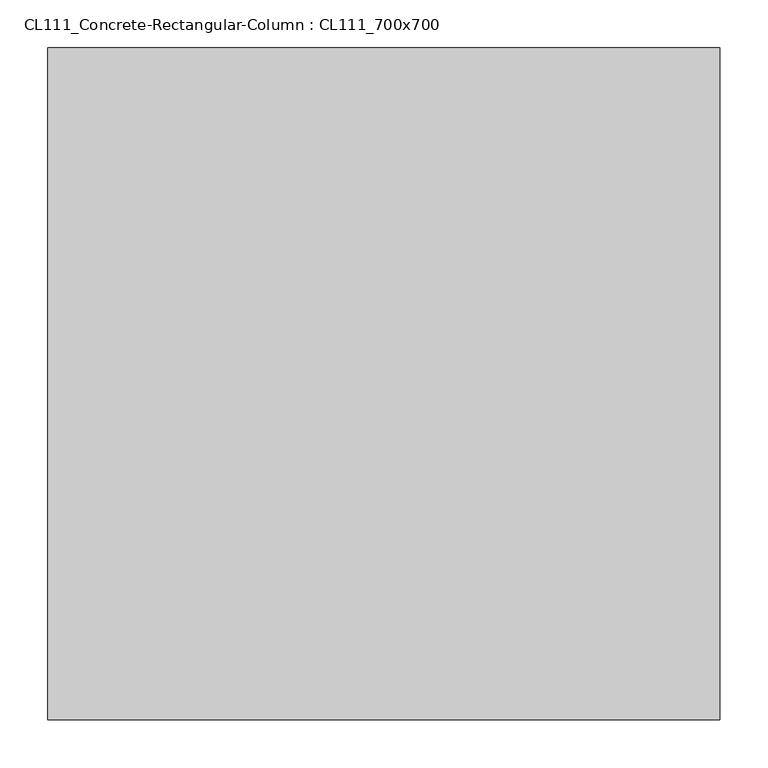
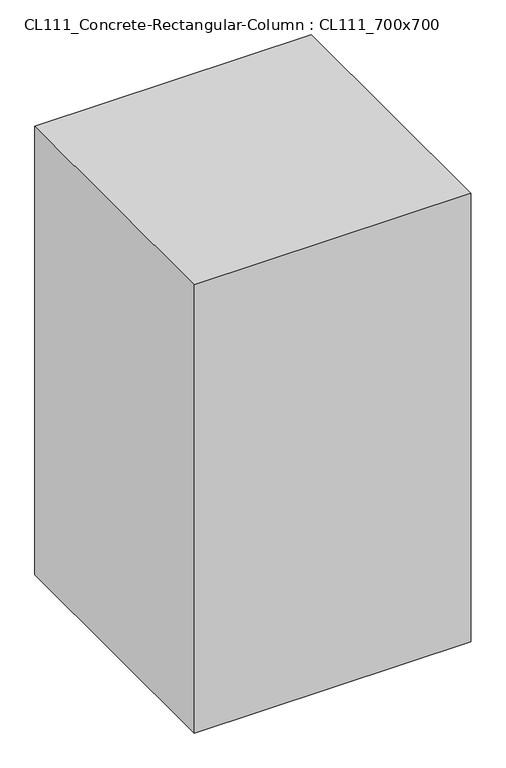
"""IFC4 building model written with IfcOpenShell, lengths in millimetres: column geometry, CL111_Concrete-Rectangular-Column : CL111_700x700."""

from ifc_helpers import new_model, si_unit, frame, origin, place, context, project, spatial, polyline, outline, extrude, source, transform, mapped, element, save


def cl111_concrete_rectangular_column_cl111_700x700_c1bab047(model_context):
    return source(origin(), model_context, "Body", "SweptSolid", [
        extrude(outline(polyline([(350.0, 350.0), (350.0, -350.0), (-350.0, -350.0), (-350.0, 350.0), (350.0, 350.0)])), frame((0.0, 0.0, -1200.0), z_axis=(0.0, 0.0, 1.0), x_axis=(1.0, 0.0, 0.0)), (0.0, 0.0, 1.0), 1200.0),
    ])


if __name__ == "__main__":
    model = new_model("IFC4")
    model_context = context("Model", 3, world=origin())
    ifc_project = project(units=[si_unit("LENGTHUNIT", "METRE", prefix="MILLI")], contexts=[model_context])
    site = spatial("IfcSite", under=ifc_project)
    building = spatial("IfcBuilding", under=site)
    placement = place(None, origin())
    cl111_concrete_rectangular_column_cl111_700x700_shape = cl111_concrete_rectangular_column_cl111_700x700_c1bab047(model_context)
    element("IfcColumn", 1, ObjectType="CL111_Concrete-Rectangular-Column : CL111_700x700", at=placement, inside=building, context=model_context, shape_type="MappedRepresentation", body=[
        mapped(cl111_concrete_rectangular_column_cl111_700x700_shape, transform((0.0, 0.0, 0.0), x_axis=(1.0, 0.0, 0.0), y_axis=(0.0, 1.0, 0.0), z_axis=(0.0, 0.0, 1.0))),
    ])
    save(model, "model.ifc")

# Revit data of these elements
# Type "CL111_Concrete-Rectangular-Column : CL111_700x700"
#   Assembly Code = "B10"
#   b = 700 mm
#   h = 700 mm
#   Structural Material [instance default] = Concrete, Cast-in-Place gray
# Element 1 (IfcColumn, "CL111_Concrete-Rectangular-Column : CL111_700x700")
#   Materials on its faces: "Concrete, Cast-in-Place gray"
# Materials
#   "Concrete, Cast-in-Place gray": class "Concrete", colour RGB 192 192 192, transparency 0, Description = "Cast-in-place concrete", Cost = 0
